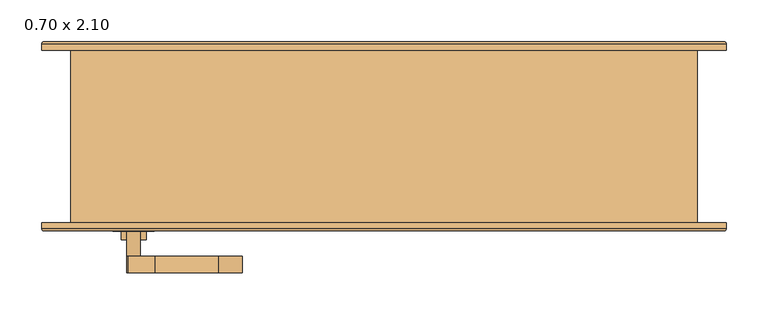
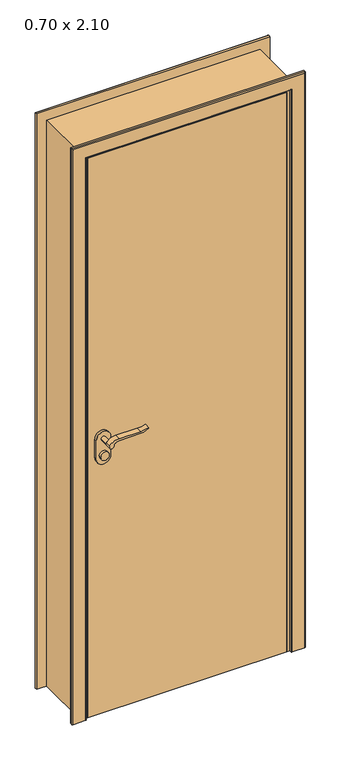
"""IFC4 building model written with IfcOpenShell, lengths in millimetres: door geometry, .CC_ND 300_PORTA SIMPLES DE ABRIR_COM EXTENSÃO : 0.70 x 2.10."""

from ifc_helpers import new_model, si_unit, point, frame, frame_2d, origin, origin_with_axes, place, context, project, spatial, polyline, circle_curve, ellipse_curve, trimmed, segment, composite_curve, outline, extrude, faceted_brep, source, transform, mapped, element, save
from ifc_brep_helpers import plane_surface, cylinder_surface, advanced_brep


def door_0_70_x_2_10_d125a7d3(model_context):
    return source(origin(), model_context, "Body", "SolidModel", [
        extrude(outline(composite_curve([segment(trimmed(circle_curve(frame_2d((964.5, -300.0)), 15.0), [point((964.5, -285.0))], [point((964.5, -315.0))], False, "CARTESIAN"), True, "CONTINUOUS"), segment(trimmed(circle_curve(frame_2d((964.5, -300.0)), 15.0), [point((964.5, -315.0))], [point((964.5, -285.0))], False, "CARTESIAN"), True, "CONTINUOUS")], self_intersect=False)), frame((0.0, -120.7, 0.0), z_axis=(0.0, 1.0, 0.0), x_axis=(0.0, 0.0, 1.0)), (0.0, 0.0, 1.0), 10.0),
        extrude(outline(composite_curve([segment(trimmed(circle_curve(frame_2d((964.5, -300.0)), 15.0), [point((964.5, -285.0))], [point((964.5, -315.0))], False, "CARTESIAN"), True, "CONTINUOUS"), segment(trimmed(circle_curve(frame_2d((964.5, -300.0)), 15.0), [point((964.5, -315.0))], [point((964.5, -285.0))], False, "CARTESIAN"), True, "CONTINUOUS")], self_intersect=False)), frame((0.0, -60.7, 0.0), z_axis=(0.0, 1.0, 0.0), x_axis=(0.0, 0.0, 1.0)), (0.0, 0.0, 1.0), 10.0),
        extrude(outline(composite_curve([segment(trimmed(circle_curve(frame_2d((1024.5, -300.0)), 8.0), [point((1029.1523287, -306.5081363))], [point((1024.5, -292.0))], False, "CARTESIAN"), True, "CONTINUOUS"), segment(trimmed(circle_curve(frame_2d((1019.3738613, -274.6138099)), 18.1261387), [point((1024.5, -292.0))], [point((1037.5, -274.6138099))], True, "CARTESIAN"), True, "CONTINUOUS"), segment(polyline([(1037.5, -274.6138099), (1037.5, -198.3564091)]), True, "CONTINUOUS"), segment(trimmed(circle_curve(frame_2d((1096.7709207, -201.9396612)), 59.3791355), [point((1037.5, -198.3564091))], [point((1046.7135558, -170.0))], False, "CARTESIAN"), True, "CONTINUOUS"), segment(polyline([(1046.7135558, -170.0), (1049.5, -170.0)]), True, "CONTINUOUS"), segment(trimmed(circle_curve(frame_2d((1127.7850638, -198.4227909)), 83.2850902), [point((1049.5, -170.0))], [point((1044.5, -198.3564091))], True, "CARTESIAN"), True, "CONTINUOUS"), segment(polyline([(1044.5, -198.3564091), (1044.5, -274.6325667)]), True, "CONTINUOUS"), segment(trimmed(circle_curve(frame_2d((1007.2555521, -276.3324871)), 37.2832219), [point((1044.5, -274.6325667))], [point((1029.1523287, -306.5081363))], False, "CARTESIAN"), True, "CONTINUOUS")], self_intersect=False)), frame((0.0, -160.7, 0.0), z_axis=(0.0, 1.0, 0.0), x_axis=(0.0, 0.0, 1.0)), (0.0, 0.0, 1.0), 20.0),
        extrude(outline(composite_curve([segment(trimmed(circle_curve(frame_2d((1019.3738682, -274.6138122)), 18.1261318), [point((1024.4999903, -292.0))], [point((1037.5, -274.6138122))], True, "CARTESIAN"), True, "CONTINUOUS"), segment(polyline([(1037.5, -274.6138122), (1037.5, -198.3564091)]), True, "CONTINUOUS"), segment(trimmed(circle_curve(frame_2d((1096.7709207, -201.9396612)), 59.3791355), [point((1037.5, -198.3564091))], [point((1046.7135558, -170.0))], False, "CARTESIAN"), True, "CONTINUOUS"), segment(polyline([(1046.7135558, -170.0), (1049.5, -170.0)]), True, "CONTINUOUS"), segment(trimmed(circle_curve(frame_2d((1127.7850638, -198.4227909)), 83.2850902), [point((1049.5, -170.0))], [point((1044.5, -198.3564091))], True, "CARTESIAN"), True, "CONTINUOUS"), segment(polyline([(1044.5, -198.3564091), (1044.5, -274.6325667)]), True, "CONTINUOUS"), segment(trimmed(circle_curve(frame_2d((1007.2555521, -276.3324871)), 37.2832219), [point((1044.5, -274.6325667))], [point((1029.1523287, -306.5081363))], False, "CARTESIAN"), True, "CONTINUOUS"), segment(trimmed(circle_curve(frame_2d((1024.5, -300.0)), 8.0), [point((1029.1523287, -306.5081363))], [point((1024.4999903, -292.0))], False, "CARTESIAN"), True, "CONTINUOUS")], self_intersect=False)), frame((0.0, -30.7, 0.0), z_axis=(0.0, 1.0, 0.0), x_axis=(0.0, 0.0, 1.0)), (0.0, 0.0, 1.0), 20.0),
        extrude(outline(composite_curve([segment(trimmed(circle_curve(frame_2d((1024.5, -300.0)), 8.0), [point((1024.5, -292.0))], [point((1024.5, -308.0))], False, "CARTESIAN"), True, "CONTINUOUS"), segment(trimmed(circle_curve(frame_2d((1024.5, -300.0)), 8.0), [point((1024.5, -308.0))], [point((1024.5, -292.0))], False, "CARTESIAN"), True, "CONTINUOUS")], self_intersect=False)), frame((0.0, -140.7, 0.0), z_axis=(0.0, 1.0, 0.0), x_axis=(0.0, 0.0, 1.0)), (0.0, 0.0, 1.0), 30.0),
        extrude(outline(composite_curve([segment(trimmed(circle_curve(frame_2d((1024.5, -300.0)), 8.0), [point((1024.5, -292.0))], [point((1024.5, -308.0))], False, "CARTESIAN"), True, "CONTINUOUS"), segment(trimmed(circle_curve(frame_2d((1024.5, -300.0)), 8.0), [point((1024.5, -308.0))], [point((1024.5, -292.0))], False, "CARTESIAN"), True, "CONTINUOUS")], self_intersect=False)), frame((0.0, -60.7, 0.0), z_axis=(0.0, 1.0, 0.0), x_axis=(0.0, 0.0, 1.0)), (0.0, 0.0, 1.0), 30.0),
        extrude(outline(composite_curve([segment(trimmed(circle_curve(frame_2d((954.5, -300.0)), 25.0), [point((954.5, -325.0))], [point((954.5, -275.0))], False, "CARTESIAN"), True, "CONTINUOUS"), segment(polyline([(954.5, -275.0), (1024.5, -275.0)]), True, "CONTINUOUS"), segment(trimmed(circle_curve(frame_2d((1024.5, -300.0)), 25.0), [point((1024.5, -275.0))], [point((1024.5, -325.0))], False, "CARTESIAN"), True, "CONTINUOUS"), segment(polyline([(1024.5, -325.0), (954.5, -325.0)]), True, "CONTINUOUS")], self_intersect=False)), frame((0.0, -110.7, 0.0), z_axis=(0.0, 1.0, 0.0), x_axis=(0.0, 0.0, 1.0)), (0.0, 0.0, 1.0), 10.0),
        extrude(outline(composite_curve([segment(trimmed(circle_curve(frame_2d((954.5, -300.0)), 25.0), [point((954.5, -325.0))], [point((954.5, -275.0))], False, "CARTESIAN"), True, "CONTINUOUS"), segment(polyline([(954.5, -275.0), (1024.5, -275.0)]), True, "CONTINUOUS"), segment(trimmed(circle_curve(frame_2d((1024.5, -300.0)), 25.0), [point((1024.5, -275.0))], [point((1024.5, -325.0))], False, "CARTESIAN"), True, "CONTINUOUS"), segment(polyline([(1024.5, -325.0), (954.5, -325.0)]), True, "CONTINUOUS")], self_intersect=False)), frame((0.0, -70.7, 0.0), z_axis=(0.0, 1.0, 0.0), x_axis=(0.0, 0.0, 1.0)), (0.0, 0.0, 1.0), 10.0),
        advanced_brep(
        [(-410.0, -100.7, 0.0), (-360.0, -100.7, 0.0), (-360.0, -107.7, 0.0), (-363.0, -110.7, 0.0), (-407.0, -110.7, 0.0), (-410.0, -107.7, 0.0), (-410.0, -100.7, 2135.0), (410.0, -100.7, 2135.0), (410.0, -100.7, 0.0), (360.0, -100.7, 0.0), (360.0, -100.7, 2085.0), (-360.0, -100.7, 2085.0), (-360.0, -107.7, 2085.0), (-363.0, -110.7, 2088.0), (363.0, -110.7, 2088.0), (363.0, -110.7, 0.0), (407.0, -110.7, 0.0), (407.0, -110.7, 2132.0), (-407.0, -110.7, 2132.0), (-410.0, -107.7, 2135.0), (410.0, -107.7, 2135.0), (410.0, -107.7, 0.0), (360.0, -107.7, 0.0), (360.0, -107.7, 2085.0)],
        [
            (0, 1),
            (1, 2),
            (2, 3, circle_curve(frame((-363.0, -107.7, 0.0), z_axis=(0.0, 0.0, -1.0), x_axis=(1.0, 0.0, 0.0)), 3.0)),
            (3, 4),
            (4, 5, circle_curve(frame((-407.0, -107.7, 0.0), z_axis=(0.0, 0.0, -1.0), x_axis=(1.0, 0.0, 0.0)), 3.0)),
            (5, 0),
            (0, 6),
            (6, 7),
            (7, 8),
            (8, 9),
            (9, 10),
            (10, 11),
            (11, 1),
            (11, 12),
            (12, 2),
            (12, 13, ellipse_curve(frame((-363.0, -107.7, 2088.0), z_axis=(-0.7071067811865475, 0.0, -0.7071067811865475), x_axis=(0.7071067811865474, 0.0, -0.7071067811865476)), 4.2426407, 3.0)),
            (13, 3),
            (13, 14),
            (14, 15),
            (15, 16),
            (16, 17),
            (17, 18),
            (18, 4),
            (18, 19, ellipse_curve(frame((-407.0, -107.7, 2132.0), z_axis=(-0.7071067811865475, 0.0, -0.7071067811865475), x_axis=(0.7071067811865474, 0.0, -0.7071067811865476)), 4.2426407, 3.0)),
            (19, 5),
            (19, 6),
            (7, 20),
            (20, 21),
            (21, 8),
            (21, 16, circle_curve(frame((407.0, -107.7, 0.0), z_axis=(0.0, 0.0, -1.0), x_axis=(-1.0, 0.0, 0.0)), 3.0)),
            (15, 22, circle_curve(frame((363.0, -107.7, 0.0), z_axis=(0.0, 0.0, -1.0), x_axis=(-1.0, 0.0, 0.0)), 3.0)),
            (22, 9),
            (23, 10),
            (22, 23),
            (14, 23, ellipse_curve(frame((363.0, -107.7, 2088.0), z_axis=(0.7071067811865475, 0.0, -0.7071067811865475), x_axis=(0.7071067811865474, 0.0, 0.7071067811865476)), 4.2426407, 3.0)),
            (20, 17, ellipse_curve(frame((407.0, -107.7, 2132.0), z_axis=(0.7071067811865475, 0.0, -0.7071067811865475), x_axis=(0.7071067811865474, 0.0, 0.7071067811865476)), 4.2426407, 3.0)),
            (23, 12),
            (19, 20),
        ],
        [
            plane_surface(frame((-360.0, -100.7, 0.0), z_axis=(0.0, 0.0, -1.0), x_axis=(0.0, 1.0, 0.0))),
            plane_surface(frame((-410.0, -100.7, 0.0), z_axis=(0.0, 1.0, 0.0), x_axis=(0.0, 0.0, 1.0))),
            plane_surface(frame((-360.0, -100.7, 0.0), z_axis=(1.0, 0.0, 0.0), x_axis=(0.0, 0.0, 1.0))),
            cylinder_surface(frame((-363.0, -107.7, 0.0), z_axis=(0.0, 0.0, -1.0), x_axis=(1.0, 0.0, 0.0)), 3.0),
            plane_surface(frame((-363.0, -110.7, 0.0), z_axis=(0.0, -1.0, 0.0), x_axis=(0.0, 0.0, 1.0))),
            cylinder_surface(frame((-407.0, -107.7, 0.0), z_axis=(0.0, 0.0, -1.0), x_axis=(1.0, 0.0, 0.0)), 3.0),
            plane_surface(frame((-410.0, -107.7, 0.0), z_axis=(-1.0, 0.0, 0.0), x_axis=(0.0, 0.0, 1.0))),
            plane_surface(frame((410.0, -107.7, 2135.0), z_axis=(1.0, 0.0, 0.0), x_axis=(0.0, 0.0, -1.0))),
            plane_surface(frame((360.0, -100.7, 0.0), z_axis=(0.0, 0.0, -1.0), x_axis=(0.0, 1.0, 0.0))),
            plane_surface(frame((360.0, -100.7, 2085.0), z_axis=(-1.0, 0.0, 0.0), x_axis=(0.0, 0.0, -1.0))),
            cylinder_surface(frame((363.0, -107.7, 2085.0), z_axis=(0.0, 0.0, 1.0), x_axis=(-1.0, 0.0, 0.0)), 3.0),
            cylinder_surface(frame((407.0, -107.7, 2085.0), z_axis=(0.0, 0.0, 1.0), x_axis=(-1.0, 0.0, 0.0)), 3.0),
            plane_surface(frame((-360.0, -100.7, 2085.0), z_axis=(0.0, 0.0, -1.0), x_axis=(1.0, 0.0, 0.0))),
            plane_surface(frame((-410.0, -107.7, 2135.0), z_axis=(0.0, 0.0, 1.0), x_axis=(1.0, 0.0, 0.0))),
            cylinder_surface(frame((-360.0, -107.7, 2088.0), z_axis=(-1.0, 0.0, 0.0), x_axis=(0.0, 0.0, -1.0)), 3.0),
            cylinder_surface(frame((-360.0, -107.7, 2132.0), z_axis=(-1.0, 0.0, 0.0), x_axis=(0.0, 0.0, -1.0)), 3.0),
        ],
        [
            (0, [[1, 2, 3, 4, 5, 6]]),
            (1, [[-1, 7, 8, 9, 10, 11, 12, 13]]),
            (2, [[-2, -13, 14, 15]]),
            (3, [[-3, -15, 16, 17]]),
            (4, [[-4, -17, 18, 19, 20, 21, 22, 23]]),
            (5, [[-5, -23, 24, 25]]),
            (6, [[-6, -25, 26, -7]]),
            (7, [[27, 28, 29, -9]]),
            (8, [[-29, 30, -20, 31, 32, -10]]),
            (9, [[33, -11, -32, 34]]),
            (10, [[35, -34, -31, -19]]),
            (11, [[36, -21, -30, -28]]),
            (12, [[-14, -12, -33, 37]]),
            (13, [[-26, 38, -27, -8]]),
            (14, [[-16, -37, -35, -18]]),
            (15, [[-24, -22, -36, -38]]),
        ],
    ),
        advanced_brep(
        [(410.0, 106.0, 0.0), (360.0, 106.0, 0.0), (360.0, 113.0157283, 0.0), (362.9842717, 116.0, 0.0), (407.0342217, 116.0, 0.0), (410.0, 113.0342217, 0.0), (410.0, 106.0, 2135.0), (-410.0, 106.0, 2135.0), (-410.0, 106.0, 0.0), (-360.0, 106.0, 0.0), (-360.0, 106.0, 2085.0), (360.0, 106.0, 2085.0), (360.0, 113.0157283, 2085.0), (362.9842717, 116.0, 2087.9842717), (-362.9842717, 116.0, 2087.9842717), (-362.9842717, 116.0, 0.0), (-407.0342217, 116.0, 0.0), (-407.0342217, 116.0, 2132.0342217), (407.0342217, 116.0, 2132.0342217), (410.0, 113.0342217, 2135.0), (-410.0, 113.0342217, 2135.0), (-410.0, 113.0342217, 0.0), (-360.0, 113.0157283, 0.0), (-360.0, 113.0157283, 2085.0)],
        [
            (0, 1),
            (1, 2),
            (2, 3, circle_curve(frame((362.9842717, 113.0157283, 0.0), z_axis=(0.0, 0.0, -1.0), x_axis=(1.0, 0.0, 0.0)), 2.9842717)),
            (3, 4),
            (4, 5, circle_curve(frame((407.0342217, 113.0342217, 0.0), z_axis=(0.0, 0.0, -1.0), x_axis=(1.0, 0.0, 0.0)), 2.9657783)),
            (5, 0),
            (0, 6),
            (6, 7),
            (7, 8),
            (8, 9),
            (9, 10),
            (10, 11),
            (11, 1),
            (11, 12),
            (12, 2),
            (12, 13, ellipse_curve(frame((362.9842717, 113.0157283, 2087.9842717), z_axis=(0.7071067811865475, 0.0, -0.7071067811865475), x_axis=(-0.7071067811865474, 0.0, -0.7071067811865476)), 4.2203975, 2.9842717)),
            (13, 3),
            (13, 14),
            (14, 15),
            (15, 16),
            (16, 17),
            (17, 18),
            (18, 4),
            (18, 19, ellipse_curve(frame((407.0342217, 113.0342217, 2132.0342217), z_axis=(0.7071067811865475, 0.0, -0.7071067811865475), x_axis=(-0.7071067811865474, 0.0, -0.7071067811865476)), 4.1942438, 2.9657783)),
            (19, 5),
            (19, 6),
            (7, 20),
            (20, 21),
            (21, 8),
            (21, 16, circle_curve(frame((-407.0342217, 113.0342217, 0.0), z_axis=(0.0, 0.0, -1.0), x_axis=(-1.0, 0.0, 0.0)), 2.9657783)),
            (15, 22, circle_curve(frame((-362.9842717, 113.0157283, 0.0), z_axis=(0.0, 0.0, -1.0), x_axis=(-1.0, 0.0, 0.0)), 2.9842717)),
            (22, 9),
            (23, 10),
            (22, 23),
            (14, 23, ellipse_curve(frame((-362.9842717, 113.0157283, 2087.9842717), z_axis=(-0.7071067811865475, 0.0, -0.7071067811865475), x_axis=(-0.7071067811865474, 0.0, 0.7071067811865476)), 4.2203975, 2.9842717)),
            (20, 17, ellipse_curve(frame((-407.0342217, 113.0342217, 2132.0342217), z_axis=(-0.7071067811865475, 0.0, -0.7071067811865475), x_axis=(-0.7071067811865474, 0.0, 0.7071067811865476)), 4.1942438, 2.9657783)),
            (23, 12),
            (19, 20),
        ],
        [
            plane_surface(frame((360.0, 106.0, 0.0), z_axis=(0.0, 0.0, -1.0), x_axis=(0.0, 1.0, 0.0))),
            plane_surface(frame((410.0, 106.0, 0.0), z_axis=(0.0, -1.0, 0.0), x_axis=(0.0, 0.0, 1.0))),
            plane_surface(frame((360.0, 106.0, 0.0), z_axis=(-1.0, 0.0, 0.0), x_axis=(0.0, 0.0, 1.0))),
            cylinder_surface(frame((362.9842717, 113.0157283, 0.0), z_axis=(0.0, 0.0, -1.0), x_axis=(1.0, 0.0, 0.0)), 2.9842717),
            plane_surface(frame((362.9842717, 116.0, 0.0), z_axis=(0.0, 1.0, 0.0), x_axis=(0.0, 0.0, 1.0))),
            cylinder_surface(frame((407.0342217, 113.0342217, 0.0), z_axis=(0.0, 0.0, -1.0), x_axis=(1.0, 0.0, 0.0)), 2.9657783),
            plane_surface(frame((410.0, 113.0342217, 0.0), z_axis=(1.0, 0.0, 0.0), x_axis=(0.0, 0.0, 1.0))),
            plane_surface(frame((-410.0, 113.0342217, 2135.0), z_axis=(-1.0, 0.0, 0.0), x_axis=(0.0, 0.0, -1.0))),
            plane_surface(frame((-360.0, 106.0, 0.0), z_axis=(0.0, 0.0, -1.0), x_axis=(0.0, 1.0, 0.0))),
            plane_surface(frame((-360.0, 106.0, 2085.0), z_axis=(1.0, 0.0, 0.0), x_axis=(0.0, 0.0, -1.0))),
            cylinder_surface(frame((-362.9842717, 113.0157283, 2085.0), z_axis=(0.0, 0.0, 1.0), x_axis=(-1.0, 0.0, 0.0)), 2.9842717),
            cylinder_surface(frame((-407.0342217, 113.0342217, 2085.0), z_axis=(0.0, 0.0, 1.0), x_axis=(-1.0, 0.0, 0.0)), 2.9657783),
            plane_surface(frame((360.0, 106.0, 2085.0), z_axis=(0.0, 0.0, -1.0), x_axis=(-1.0, 0.0, 0.0))),
            plane_surface(frame((410.0, 113.0342217, 2135.0), z_axis=(0.0, 0.0, 1.0), x_axis=(-1.0, 0.0, 0.0))),
            cylinder_surface(frame((360.0, 113.0157283, 2087.9842717), z_axis=(1.0, 0.0, 0.0), x_axis=(0.0, 0.0, 1.0)), 2.9842717),
            cylinder_surface(frame((360.0, 113.0342217, 2132.0342217), z_axis=(1.0, 0.0, 0.0), x_axis=(0.0, 0.0, 1.0)), 2.9657783),
        ],
        [
            (0, [[1, 2, 3, 4, 5, 6]]),
            (1, [[-1, 7, 8, 9, 10, 11, 12, 13]]),
            (2, [[-2, -13, 14, 15]]),
            (3, [[-3, -15, 16, 17]]),
            (4, [[-4, -17, 18, 19, 20, 21, 22, 23]]),
            (5, [[-5, -23, 24, 25]]),
            (6, [[-6, -25, 26, -7]]),
            (7, [[27, 28, 29, -9]]),
            (8, [[-29, 30, -20, 31, 32, -10]]),
            (9, [[33, -11, -32, 34]]),
            (10, [[35, -34, -31, -19]]),
            (11, [[36, -21, -30, -28]]),
            (12, [[-14, -12, -33, 37]]),
            (13, [[-26, 38, -27, -8]]),
            (14, [[-16, -37, -35, -18]]),
            (15, [[-24, -22, -36, -38]]),
        ],
    ),
        faceted_brep([(342.0, 106.0, 0.0), (375.0, 106.0, 0.0), (375.0, -100.7, 0.0), (350.0, -100.7, 0.0), (350.0, -70.7, 0.0), (342.0, -70.7, 0.0), (342.0, 106.0, 2067.0), (-342.0, 106.0, 2067.0), (-342.0, 106.0, 0.0), (-375.0, 106.0, 0.0), (-375.0, 106.0, 2100.0), (375.0, 106.0, 2100.0), (375.0, -100.7, 2100.0), (-375.0, -100.7, 2100.0), (-375.0, -100.7, 0.0), (-350.0, -100.7, 0.0), (-350.0, -100.7, 2075.0), (350.0, -100.7, 2075.0), (350.0, -70.7, 2075.0), (-350.0, -70.7, 2075.0), (-350.0, -70.7, 0.0), (-342.0, -70.7, 0.0), (-342.0, -70.7, 2067.0), (342.0, -70.7, 2067.0)], [[[0, 1, 2, 3, 4, 5]], [[1, 0, 6, 7, 8, 9, 10, 11]], [[2, 1, 11, 12]], [[3, 2, 12, 13, 14, 15, 16, 17]], [[4, 3, 17, 18]], [[5, 4, 18, 19, 20, 21, 22, 23]], [[0, 5, 23, 6]], [[7, 22, 21, 8]], [[8, 21, 20, 15, 14, 9]], [[13, 10, 9, 14]], [[19, 16, 15, 20]], [[12, 11, 10, 13]], [[18, 17, 16, 19]], [[6, 23, 22, 7]]]),
        extrude(outline(polyline([(-350.0, -70.7), (350.0, -70.7), (350.0, -100.7), (-350.0, -100.7), (-350.0, -70.7)])), origin_with_axes(), (0.0, 0.0, 1.0), 2075.0),
    ])


if __name__ == "__main__":
    model = new_model("IFC4")
    model_context = context("Model", 3, world=origin())
    ifc_project = project(units=[si_unit("LENGTHUNIT", "METRE", prefix="MILLI")], contexts=[model_context])
    site = spatial("IfcSite", under=ifc_project)
    building = spatial("IfcBuilding", under=site)
    placement = place(None, origin())
    door_0_70_x_2_10_shape = door_0_70_x_2_10_d125a7d3(model_context)
    element("IfcDoor", 1, ObjectType=".CC_ND 300_PORTA SIMPLES DE ABRIR_COM EXTENSÃO : 0.70 x 2.10", at=placement, inside=building, context=model_context, shape_type="MappedRepresentation", body=[
        mapped(door_0_70_x_2_10_shape, transform((0.0, 0.0, 0.0), x_axis=(1.0, 0.0, 0.0), y_axis=(0.0, 1.0, 0.0), z_axis=(0.0, 0.0, 1.0))),
    ])
    save(model, "model.ifc")

# Revit data of these elements
# Type ".CC_ND 300_PORTA SIMPLES DE ABRIR_COM EXTENSÃO : 0.70 x 2.10"
#   Type Mark = "155"
#   Rough Width = 0.75 m
#   Espessura moldura externa = 0.01 m
#   Espessura moldura interna = 0.01 m
#   Largura moldura = 0.05 m
#   Extensão acabamento exterior [instance default] = 0.00 m
#   Extensão acabamento interior [instance default] = 0.00 m
#   Espessura batente = 0.025 m
#   Thickness = 0.03 m
#   Altura batente = 2.085 m
#   Aux Arco [instance default] = 0.70 m
#   Rough Height = 2.125 m
#   Height = 2.10 m
#   Width = 0.70 m
#   Moldura interna [instance default] = yes
#   Moldura externa [instance default] = yes
#   Porta = .MADEIRA COM PINTURA ESMALTE BRANCO ACETINADO
#   Moldura = .MADEIRA COM PINTURA ESMALTE BRANCO ACETINADO
#   Maçaneta = .ALUMÍNIO
#   Batente = .MADEIRA COM PINTURA ESMALTE BRANCO ACETINADO
#   Function = (empty or 0)
#   Wall Closure = (empty or 0)
# Element 1 (IfcDoor, ".CC_ND 300_PORTA SIMPLES DE ABRIR_COM EXTENSÃO : 0.70 x 2.10")
#   Extensão acabamento exterior = 0.031 m
#   Extensão acabamento interior = 0.0257 m
#   Aux Arco = 0.7257 m
#   Materials on its faces: ".MADEIRA COM PINTURA ESMALTE BRANCO ACETINADO", ".ALUMÍNIO"
# Materials
#   ".MADEIRA COM PINTURA ESMALTE BRANCO ACETINADO": class ".CC_MADEIRAS", colour RGB 240 240 240, transparency 0, Description = "Madeira com pintura esmalte branco acetinado.", Cost = 0
#   ".ALUMÍNIO": class "CC_METAIS", colour RGB 244 244 244, transparency 0, Description = "Material alumínio", Cost = 0
